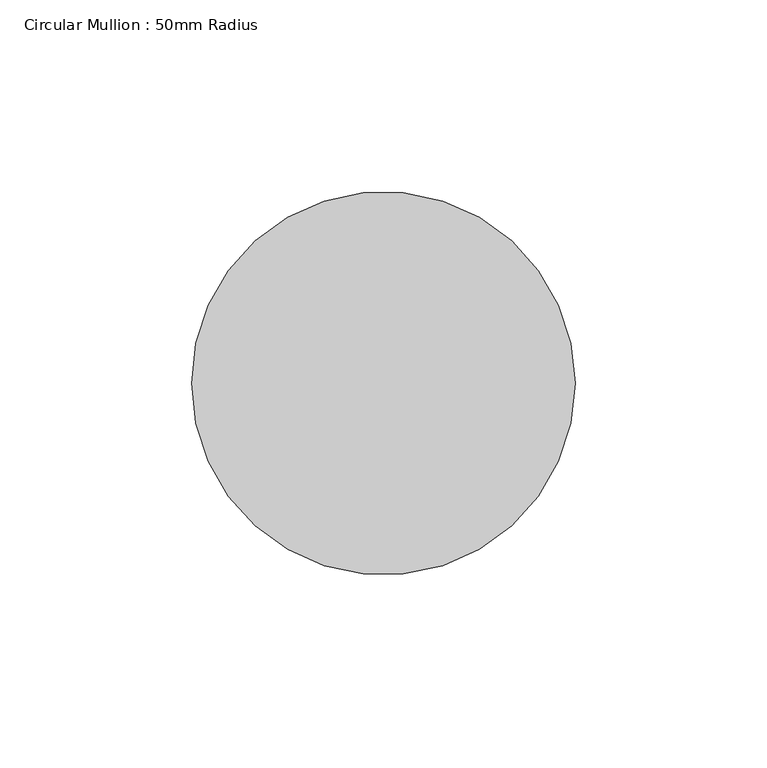
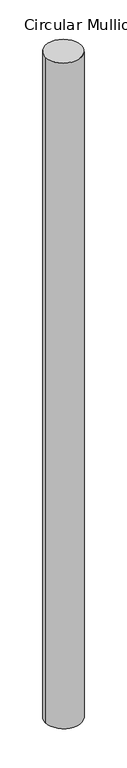
"""IFC4 building model written with IfcOpenShell, lengths in millimetres: member geometry, Circular Mullion : 50mm Radius."""

from ifc_helpers import new_model, si_unit, point, frame, origin, origin_2d, place, context, project, spatial, circle_curve, trimmed, segment, composite_curve, outline, extrude, source, transform, mapped, element, save


def circular_mullion_50mm_radius_c9b9977d(model_context):
    return source(origin(), model_context, "Body", "SweptSolid", [
        extrude(outline(composite_curve([segment(trimmed(circle_curve(origin_2d(), 50.0), [point((50.0, 0.0))], [point((-50.0, 0.0))], False, "CARTESIAN"), True, "CONTINUOUS"), segment(trimmed(circle_curve(origin_2d(), 50.0), [point((-50.0, 0.0))], [point((50.0, 0.0))], False, "CARTESIAN"), True, "CONTINUOUS")], self_intersect=False)), frame((0.0, 0.0, -1953.9783701), z_axis=(0.0, 0.0, 1.0), x_axis=(1.0, 0.0, 0.0)), (0.0, 0.0, 1.0), 1953.9783701),
    ])


if __name__ == "__main__":
    model = new_model("IFC4")
    model_context = context("Model", 3, world=origin())
    ifc_project = project(units=[si_unit("LENGTHUNIT", "METRE", prefix="MILLI")], contexts=[model_context])
    site = spatial("IfcSite", under=ifc_project)
    building = spatial("IfcBuilding", under=site)
    placement = place(None, origin())
    circular_mullion_50mm_radius_shape = circular_mullion_50mm_radius_c9b9977d(model_context)
    element("IfcMember", 1, ObjectType="Circular Mullion : 50mm Radius", at=placement, inside=building, context=model_context, shape_type="MappedRepresentation", body=[
        mapped(circular_mullion_50mm_radius_shape, transform((0.0, 0.0, 0.0), x_axis=(1.0, 0.0, 0.0), y_axis=(0.0, 1.0, 0.0), z_axis=(0.0, 0.0, 1.0))),
    ])
    save(model, "model.ifc")

# Revit data of these elements
# Type "Circular Mullion : 50mm Radius"
#   built-in parameter 1007350 = 0.164042 (stored number, unit not read)
# Element 1 (IfcMember, "Circular Mullion : 50mm Radius")
#   Materials on its faces: "Aluminium"
# Materials
#   "Aluminium": class "Metal", colour RGB 247 247 247, transparency 0, Description = "Aluminium 6061", Cost = 0
